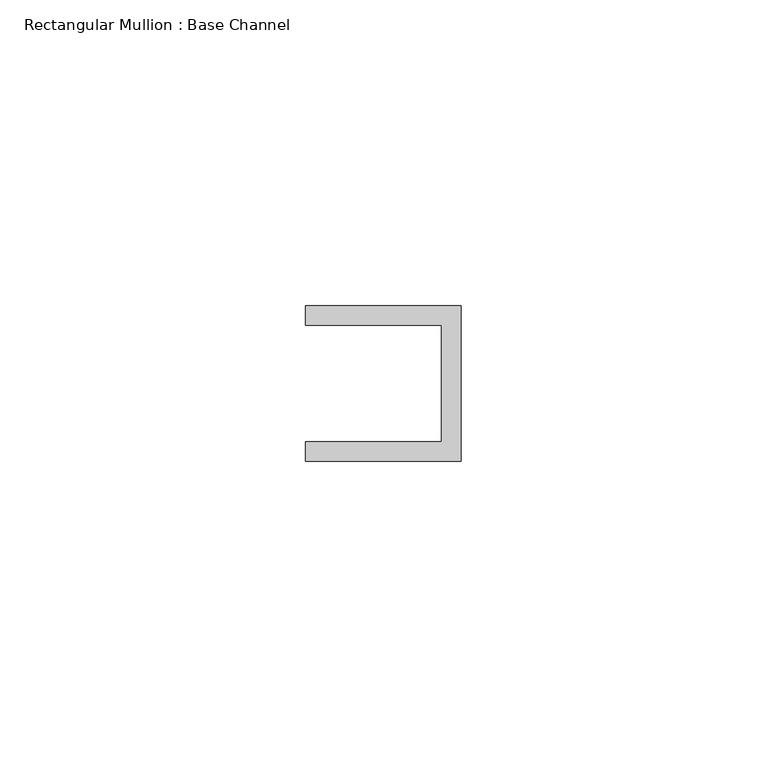
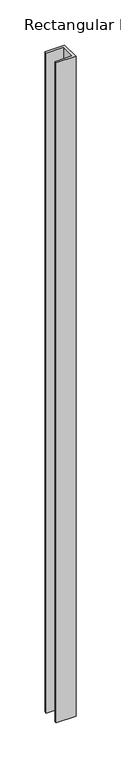
"""IFC4 building model written with IfcOpenShell, lengths in millimetres: member geometry, Rectangular Mullion : Base Channel."""

from ifc_helpers import new_model, si_unit, frame, origin, place, context, project, spatial, polyline, outline, extrude, source, transform, mapped, element, save


def rectangular_mullion_base_channel_f6e6cf7c(model_context):
    return source(origin(), model_context, "Body", "SweptSolid", [
        extrude(outline(polyline([(0.0, -12.7), (-25.4, -12.7), (-25.4, -9.525), (-3.175, -9.525), (-3.175, 9.525), (-25.4, 9.525), (-25.4, 12.7), (0.0, 12.7), (0.0, -12.7)])), frame((0.0, 0.0, -894.320152), z_axis=(0.0, 0.0, 1.0), x_axis=(1.0, 0.0, 0.0)), (0.0, 0.0, 1.0), 894.320152),
    ])


if __name__ == "__main__":
    model = new_model("IFC4")
    model_context = context("Model", 3, world=origin())
    ifc_project = project(units=[si_unit("LENGTHUNIT", "METRE", prefix="MILLI")], contexts=[model_context])
    site = spatial("IfcSite", under=ifc_project)
    building = spatial("IfcBuilding", under=site)
    placement = place(None, origin())
    rectangular_mullion_base_channel_shape = rectangular_mullion_base_channel_f6e6cf7c(model_context)
    element("IfcMember", 1, ObjectType="Rectangular Mullion : Base Channel", at=placement, inside=building, context=model_context, shape_type="MappedRepresentation", body=[
        mapped(rectangular_mullion_base_channel_shape, transform((0.0, 0.0, 0.0), x_axis=(1.0, 0.0, 0.0), y_axis=(0.0, 1.0, 0.0), z_axis=(0.0, 0.0, 1.0))),
    ])
    save(model, "model.ifc")

# Revit data of these elements
# Type "Rectangular Mullion : Base Channel"
#   built-in parameter 1007322 = 0.0833333 (stored number, unit not read)
#   built-in parameter 1007321 = 0.0416667 (stored number, unit not read)
#   built-in parameter 1007320 = -0.03125 (stored number, unit not read)
# Element 1 (IfcMember, "Rectangular Mullion : Base Channel")
#   Materials on its faces: "ALUM"
# Materials
#   "ALUM": class "Generic", colour RGB 157 157 157, transparency 0, Cost = 0
